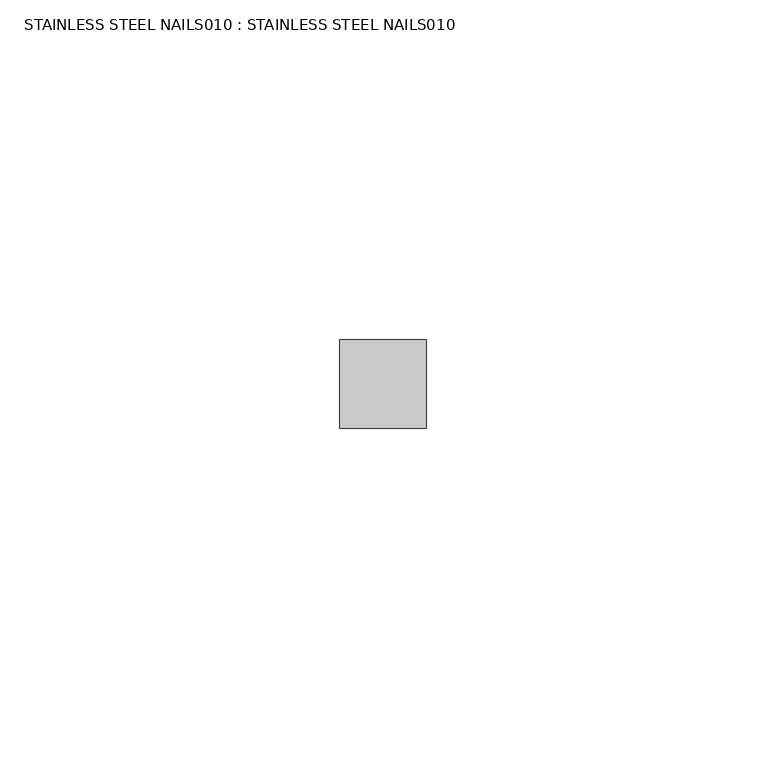
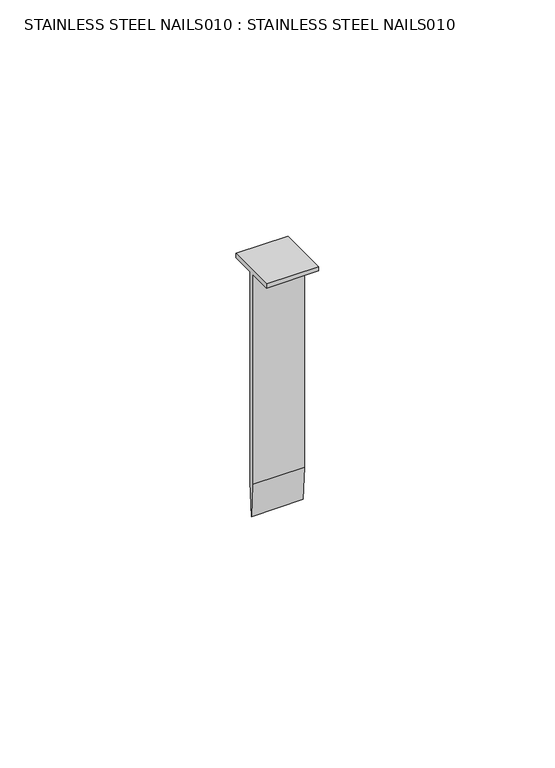
"""IFC4 building model written with IfcOpenShell, lengths in millimetres: proxy geometry, STAINLESS STEEL NAILS010 : STAINLESS STEEL NAILS010."""

from ifc_helpers import new_model, si_unit, frame, origin, place, context, project, spatial, polyline, outline, extrude, source, transform, mapped, element, save


def stainless_steel_nails010_stainless_steel_nails010_4bc19ad7(model_context):
    return source(origin(), model_context, "Body", "SweptSolid", [
        extrude(outline(polyline([(-5473.1767457, 40241.4271837), (-5473.1767457, 40242.5103824), (-5460.1783618, 40242.5103824), (-5460.1783618, 40241.4271837), (-5466.1359544, 40241.4271837), (-5466.1359544, 40187.1002906), (-5466.6775537, 40178.4347014), (-5467.2191531, 40187.1002906), (-5467.2191531, 40241.4271837), (-5473.1767457, 40241.4271837)])), frame((14383.0178845, 0.0, 0.0), z_axis=(1.0, 0.0, 0.0), x_axis=(0.0, 1.0, 0.0)), (0.0, 0.0, 1.0), 12.7),
    ])


if __name__ == "__main__":
    model = new_model("IFC4")
    model_context = context("Model", 3, world=origin())
    ifc_project = project(units=[si_unit("LENGTHUNIT", "METRE", prefix="MILLI")], contexts=[model_context])
    site = spatial("IfcSite", under=ifc_project)
    building = spatial("IfcBuilding", under=site)
    placement = place(None, origin())
    stainless_steel_nails010_stainless_steel_nails010_shape = stainless_steel_nails010_stainless_steel_nails010_4bc19ad7(model_context)
    element("IfcBuildingElementProxy", 1, Name="STAINLESS STEEL NAILS010 : STAINLESS STEEL NAILS010", ObjectType="STAINLESS STEEL NAILS010 : STAINLESS STEEL NAILS010", at=placement, inside=building, context=model_context, shape_type="MappedRepresentation", body=[
        mapped(stainless_steel_nails010_stainless_steel_nails010_shape, transform((0.0, 0.0, 0.0), x_axis=(1.0, 0.0, 0.0), y_axis=(0.0, 1.0, 0.0), z_axis=(0.0, 0.0, 1.0))),
    ])
    save(model, "model.ifc")

# Revit data of these elements
# Type "STAINLESS STEEL NAILS010 : STAINLESS STEEL NAILS010"
#   NameOverride = "STAINLESS STEEL NAILS010"
# Element 1 (IfcBuildingElementProxy, "STAINLESS STEEL NAILS010 : STAINLESS STEEL NAILS010")
#   Materials on its faces: "1 3/4\" STAINLESS STEEL RINGSHANK 5D COMMON NAILS @ 4\" (101.6MM) O.C. FIRESTONE PROVIDED MAX., 1/2\" STAGGERED"
# Materials
#   "1 3/4\" STAINLESS STEEL RINGSHANK 5D COMMON NAILS @ 4\" (101.6MM) O.C. FIRESTONE PROVIDED MAX., 1/2\" STAGGERED": class "Unassigned", colour RGB 255 255 255, transparency 0
